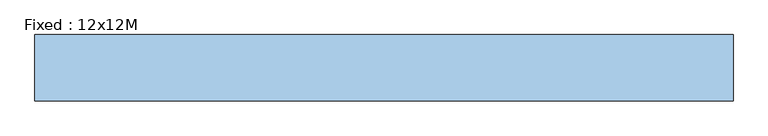
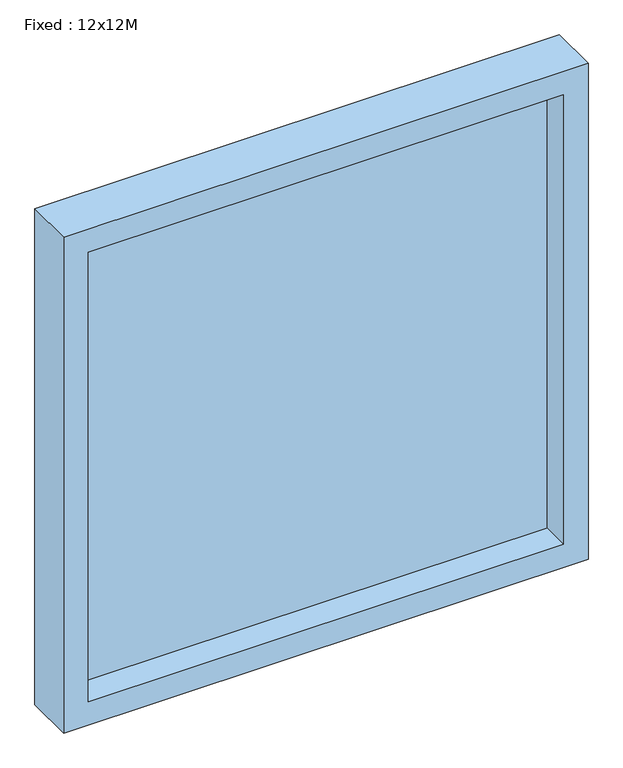
"""IFC4 building model written with IfcOpenShell, lengths in millimetres: window geometry, Fixed : 12x12M."""

import ifcopenshell
import ifcopenshell.guid

model = None  # the IFC model being written
_history = None  # IfcOwnerHistory: only IFC2X3 demands one
_inside = {}  # id of a spatial element -> (the spatial element, [elements in it])
_under = {}  # id of a project, library or spatial element -> (it, [spatial elements below it])
_declared = {}  # id of a project -> (the project, [libraries it declares])
_typed = {}  # id of a type object -> (the type object, [elements of that type])
_made_of = {}  # id of a material, layer set ... -> (it, [elements and type objects made of it])


def new_model(schema):
    """Start an empty IFC model of exactly this schema.

    Asked for "IFC4X3", IfcOpenShell would pick the latest addendum, in which some entities
    have other attributes; the version numbers below select the first issue.
    IFC2X3 requires an IfcOwnerHistory on every rooted entity: one is made here for all.
    """
    global model, _history
    if schema == "IFC4X3":
        model = ifcopenshell.file(schema_version=(4, 3, 0, 0))
    else:
        model = ifcopenshell.file(schema=schema)
    _inside.clear()
    _under.clear()
    _declared.clear()
    _typed.clear()
    _made_of.clear()
    _history = None
    if model.schema == "IFC2X3":
        org = make("IfcOrganization", Name="unknown")
        user = make(
            "IfcPersonAndOrganization",
            ThePerson=make("IfcPerson", FamilyName="unknown"),
            TheOrganization=org,
        )
        app = make(
            "IfcApplication",
            ApplicationDeveloper=org,
            Version="unknown",
            ApplicationFullName="unknown",
            ApplicationIdentifier="unknown",
        )
        _history = make(
            "IfcOwnerHistory",
            OwningUser=user,
            OwningApplication=app,
            ChangeAction="ADDED",
            CreationDate=0,
        )
    return model


def make(cls, **values):
    """One entity of the class cls with the attributes given. An attribute that is None is left unset."""
    return model.create_entity(
        cls, **{name: value for name, value in values.items() if value is not None}
    )


def rooted(cls, **values):
    """An entity with a GlobalId (a new one), such as an element, a storey or a relation."""
    return make(cls, GlobalId=ifcopenshell.guid.new(), OwnerHistory=_history, **values)


def si_unit(unit_type, name, prefix=None):
    """IfcSIUnit, for example si_unit("LENGTHUNIT", "METRE", prefix="MILLI")."""
    return make("IfcSIUnit", UnitType=unit_type, Prefix=prefix, Name=name)


def assignment(units):
    """IfcUnitAssignment: the units of a project."""
    return None if units is None else make("IfcUnitAssignment", Units=units)


def point(xyz):
    """IfcCartesianPoint."""
    return None if xyz is None else make("IfcCartesianPoint", Coordinates=xyz)


def direction(xyz):
    """IfcDirection."""
    return None if xyz is None else make("IfcDirection", DirectionRatios=xyz)


def frame(location, z_axis=None, x_axis=None):
    """IfcAxis2Placement3D, a coordinate frame: its origin and axes. An axis left out is left unset."""
    return make(
        "IfcAxis2Placement3D",
        Location=point(location),
        Axis=direction(z_axis),
        RefDirection=direction(x_axis),
    )


def origin():
    """The frame at (0, 0, 0) with its axes left unset."""
    return frame((0.0, 0.0, 0.0))


def place(relative_to, where):
    """IfcLocalPlacement: puts the frame where relative to a parent placement (None: the world)."""
    return make(
        "IfcLocalPlacement", PlacementRelTo=relative_to, RelativePlacement=where
    )


def context(
    kind, dimensions, precision=None, world=None, true_north=None, identifier=None
):
    """IfcGeometricRepresentationContext, for example the 3D "Model" context."""
    return make(
        "IfcGeometricRepresentationContext",
        ContextIdentifier=identifier,
        ContextType=kind,
        CoordinateSpaceDimension=dimensions,
        Precision=precision,
        WorldCoordinateSystem=world,
        TrueNorth=true_north,
    )


def project(units=None, contexts=None):
    """IfcProject with its units and contexts."""
    return rooted(
        "IfcProject",
        Name="project",
        RepresentationContexts=contexts,
        UnitsInContext=assignment(units),
    )


def spatial(cls, under=None, at=None, **own):
    """A site, building, storey or space (cls), placed at a placement, below another one or the project."""
    s = rooted(cls, ObjectPlacement=at, **own)
    if under is not None:
        _under.setdefault(under.id(), (under, []))[1].append(s)
    return s


def polyline(points):
    """IfcPolyline through the points."""
    return make("IfcPolyline", Points=[point(p) for p in points])


def outline(outer, holes=None, kind="AREA"):
    """IfcArbitraryClosedProfileDef: a profile drawn as a closed curve; with holes, ...WithVoids."""
    if holes is None:
        return make("IfcArbitraryClosedProfileDef", ProfileType=kind, OuterCurve=outer)
    return make(
        "IfcArbitraryProfileDefWithVoids",
        ProfileType=kind,
        OuterCurve=outer,
        InnerCurves=holes,
    )


def extrude(swept, where, along, depth):
    """IfcExtrudedAreaSolid: the profile swept, set in the frame where, extruded along a direction by depth."""
    return make(
        "IfcExtrudedAreaSolid",
        SweptArea=swept,
        Position=where,
        ExtrudedDirection=direction(along),
        Depth=depth,
    )


def shape(context_of_items, identifier, shape_type, items):
    """IfcShapeRepresentation: the items that make up one representation, for example the "Body"."""
    return make(
        "IfcShapeRepresentation",
        ContextOfItems=context_of_items,
        RepresentationIdentifier=identifier,
        RepresentationType=shape_type,
        Items=items,
    )


def source(mapping_origin, context_of_items, identifier, shape_type, items):
    """IfcRepresentationMap: a shape defined once, which mapped items show again and again."""
    return make(
        "IfcRepresentationMap",
        MappingOrigin=mapping_origin,
        MappedRepresentation=shape(context_of_items, identifier, shape_type, items),
    )


def transform(
    local_origin,
    x_axis=None,
    y_axis=None,
    z_axis=None,
    scale=None,
    scale2=None,
    scale3=None,
    uniform=True,
):
    """IfcCartesianTransformationOperator3D, or its non-uniform kind. x_axis, y_axis, z_axis: its Axis1, 2, 3."""
    if uniform:
        return make(
            "IfcCartesianTransformationOperator3D",
            Axis1=direction(x_axis),
            Axis2=direction(y_axis),
            LocalOrigin=point(local_origin),
            Scale=scale,
            Axis3=direction(z_axis),
        )
    return make(
        "IfcCartesianTransformationOperator3DnonUniform",
        Axis1=direction(x_axis),
        Axis2=direction(y_axis),
        LocalOrigin=point(local_origin),
        Scale=scale,
        Axis3=direction(z_axis),
        Scale2=scale2,
        Scale3=scale3,
    )


def mapped(mapping_source, mapping_target):
    """IfcMappedItem: shows the shape of a source again, moved by a transform."""
    return make(
        "IfcMappedItem", MappingSource=mapping_source, MappingTarget=mapping_target
    )


def made_of(thing, what):
    """Note that an element or type object is made of a material, layer set ...; save() writes the relation."""
    if what is not None:
        _made_of.setdefault(what.id(), (what, []))[1].append(thing)
    return thing


def element(
    cls,
    number,
    at=None,
    inside=None,
    cuts=None,
    type_object=None,
    material=None,
    context=None,
    identifier="Body",
    shape_type=None,
    held_by="IfcProductDefinitionShape",
    body=None,
    shapes=None,
    **own,
):
    """One element of the class cls, such as IfcWall. Its Tag is "e" and its number.

    at: its placement. inside: the storey or other place that contains it. cuts: it is an
    opening in that element (IfcRelVoidsElement). A single representation is given by context,
    identifier, shape_type and body (its items); several are given by shapes. held_by: the class
    of the entity that holds the representations. save() writes the other relations.
    """
    e = rooted(cls, Tag="e%d" % number, ObjectPlacement=at, **own)
    if body is not None:
        shapes = [shape(context, identifier, shape_type, body)]
    if shapes is not None:
        e.Representation = make(held_by, Representations=shapes)
    if inside is not None:
        _inside.setdefault(inside.id(), (inside, []))[1].append(e)
    if cuts is not None:
        rooted(
            "IfcRelVoidsElement", RelatingBuildingElement=cuts, RelatedOpeningElement=e
        )
    if type_object is not None:
        _typed.setdefault(type_object.id(), (type_object, []))[1].append(e)
    return made_of(e, material)


def aggregate(whole, parts):
    """IfcRelAggregates: a whole, such as a stair, and the parts it consists of."""
    return rooted("IfcRelAggregates", RelatingObject=whole, RelatedObjects=parts)


def save(model, path):
    """Write the relations noted so far, then the file.

    IfcRelAggregates (storeys below a building ...), IfcRelContainedInSpatialStructure (elements
    in a storey), IfcRelDefinesByType, IfcRelAssociatesMaterial and IfcRelDeclares: one each for
    every whole, place, type object, material and project.
    """
    for whole, parts in _under.values():
        aggregate(whole, parts)
    for where, things in _inside.values():
        rooted(
            "IfcRelContainedInSpatialStructure",
            RelatedElements=things,
            RelatingStructure=where,
        )
    for kind, things in _typed.values():
        rooted("IfcRelDefinesByType", RelatedObjects=things, RelatingType=kind)
    for what, things in _made_of.values():
        rooted("IfcRelAssociatesMaterial", RelatedObjects=things, RelatingMaterial=what)
    for by, libraries in _declared.values():
        rooted("IfcRelDeclares", RelatingContext=by, RelatedDefinitions=libraries)
    model.write(path)


def fixed_12x12m_54af5089(model_context):
    return source(origin(), model_context, "Body", "SweptSolid", [
        extrude(outline(polyline([(2012.0, 606.0), (2012.0, -606.0), (800.0, -606.0), (800.0, 606.0), (2012.0, 606.0)]), holes=[polyline([(857.0, 549.0), (857.0, -549.0), (1955.0, -549.0), (1955.0, 549.0), (857.0, 549.0)])]), frame((0.0, 69.0, 0.0), z_axis=(0.0, 1.0, 0.0), x_axis=(0.0, 0.0, 1.0)), (0.0, 0.0, 1.0), 115.0),
        extrude(outline(polyline([(-549.0, 162.0), (549.0, 162.0), (549.0, 134.0), (-549.0, 134.0), (-549.0, 162.0)])), frame((0.0, 0.0, 857.0), z_axis=(0.0, 0.0, 1.0), x_axis=(1.0, 0.0, 0.0)), (0.0, 0.0, 1.0), 1098.0),
    ])


if __name__ == "__main__":
    model = new_model("IFC4")
    model_context = context("Model", 3, world=origin())
    ifc_project = project(units=[si_unit("LENGTHUNIT", "METRE", prefix="MILLI")], contexts=[model_context])
    site = spatial("IfcSite", under=ifc_project)
    building = spatial("IfcBuilding", under=site)
    placement = place(None, origin())
    fixed_12x12m_shape = fixed_12x12m_54af5089(model_context)
    element("IfcWindow", 1, ObjectType="Fixed : 12x12M", at=placement, inside=building, context=model_context, shape_type="MappedRepresentation", body=[
        mapped(fixed_12x12m_shape, transform((0.0, 0.0, 0.0), x_axis=(1.0, 0.0, 0.0), y_axis=(0.0, 1.0, 0.0), z_axis=(0.0, 0.0, 1.0))),
    ])
    save(model, "model.ifc")

# Revit data of these elements
# Project information
#   Client Name = "Test Project"
#   Project Address = "Enter address here"
#   Project Number = "Number"
#   Current Version = "0.0.0"
#   SR Document GUID = "3eb9317e-835d-4f79-8926-4d15b96bc824"
# Type "Fixed : 12x12M"
#   Type Mark = "55"
#   Creator Organization [instance default] = "© Danish Educational Content"
#   Creator Name [instance default] = "© Erik Falck Jørgensen"
#   Creator Build [instance default] = "2017.0801.0"
#   Analytic Construction = "<None>"
#   length#5 = -22 mm
#   length#4 = -50 mm
#   length#3 = 100 mm
#   length#2 = 57 mm
#   length#1 = 0 mm
#   Seal Width = 12 mm
#   Rough Width = 1212 mm
#   Rough Height = 1212 mm
#   Rebate Depth = 50 mm
#   Height = 1188 mm
#   Glass Thickness = 28 mm
#   Exterior Direction [instance default] = 0.00°
#   Default Sill Height = 800 mm
#   Width = 1188 mm
#   Case Width = 45 mm
#   Case Depth = 115 mm
#   Sealing = no
#   Wall Closure = 1
#   Above Cutplane [instance default] = no
#   Wall Surface = none
#   Sill Plate = none
#   Glass = none
#   Embrasure = none
#   Case/Transom = none
#   Assembly Code = ""
# Element 1 (IfcWindow, "Fixed : 12x12M")
#   Materials on its faces: "Default Frame/Mullion (Interior/Exterior)", "Glass"
# Materials
#   "Default Frame/Mullion (Interior/Exterior)": class "Generic", colour RGB 205 205 205, transparency 0, Description = "Udefineret karm/ramme materiale", Cost = 0
#   "Glass": class "Glass", colour RGB 180 200 255, transparency 0.75, Description = "Generisk glas", Cost = 0
